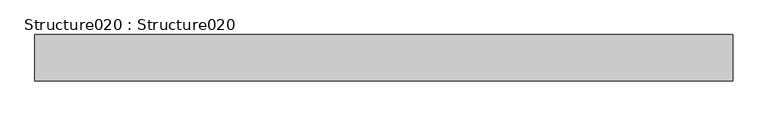
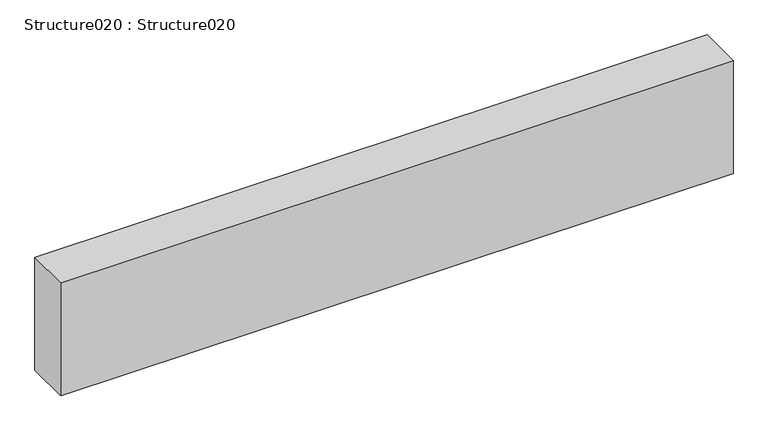
"""IFC4 building model written with IfcOpenShell, lengths in millimetres: proxy geometry, Structure020 : Structure020."""

import ifcopenshell
import ifcopenshell.guid

model = None  # the IFC model being written
_history = None  # IfcOwnerHistory: only IFC2X3 demands one
_inside = {}  # id of a spatial element -> (the spatial element, [elements in it])
_under = {}  # id of a project, library or spatial element -> (it, [spatial elements below it])
_declared = {}  # id of a project -> (the project, [libraries it declares])
_typed = {}  # id of a type object -> (the type object, [elements of that type])
_made_of = {}  # id of a material, layer set ... -> (it, [elements and type objects made of it])


def new_model(schema):
    """Start an empty IFC model of exactly this schema.

    Asked for "IFC4X3", IfcOpenShell would pick the latest addendum, in which some entities
    have other attributes; the version numbers below select the first issue.
    IFC2X3 requires an IfcOwnerHistory on every rooted entity: one is made here for all.
    """
    global model, _history
    if schema == "IFC4X3":
        model = ifcopenshell.file(schema_version=(4, 3, 0, 0))
    else:
        model = ifcopenshell.file(schema=schema)
    _inside.clear()
    _under.clear()
    _declared.clear()
    _typed.clear()
    _made_of.clear()
    _history = None
    if model.schema == "IFC2X3":
        org = make("IfcOrganization", Name="unknown")
        user = make(
            "IfcPersonAndOrganization",
            ThePerson=make("IfcPerson", FamilyName="unknown"),
            TheOrganization=org,
        )
        app = make(
            "IfcApplication",
            ApplicationDeveloper=org,
            Version="unknown",
            ApplicationFullName="unknown",
            ApplicationIdentifier="unknown",
        )
        _history = make(
            "IfcOwnerHistory",
            OwningUser=user,
            OwningApplication=app,
            ChangeAction="ADDED",
            CreationDate=0,
        )
    return model


def make(cls, **values):
    """One entity of the class cls with the attributes given. An attribute that is None is left unset."""
    return model.create_entity(
        cls, **{name: value for name, value in values.items() if value is not None}
    )


def rooted(cls, **values):
    """An entity with a GlobalId (a new one), such as an element, a storey or a relation."""
    return make(cls, GlobalId=ifcopenshell.guid.new(), OwnerHistory=_history, **values)


def si_unit(unit_type, name, prefix=None):
    """IfcSIUnit, for example si_unit("LENGTHUNIT", "METRE", prefix="MILLI")."""
    return make("IfcSIUnit", UnitType=unit_type, Prefix=prefix, Name=name)


def assignment(units):
    """IfcUnitAssignment: the units of a project."""
    return None if units is None else make("IfcUnitAssignment", Units=units)


def point(xyz):
    """IfcCartesianPoint."""
    return None if xyz is None else make("IfcCartesianPoint", Coordinates=xyz)


def direction(xyz):
    """IfcDirection."""
    return None if xyz is None else make("IfcDirection", DirectionRatios=xyz)


def frame(location, z_axis=None, x_axis=None):
    """IfcAxis2Placement3D, a coordinate frame: its origin and axes. An axis left out is left unset."""
    return make(
        "IfcAxis2Placement3D",
        Location=point(location),
        Axis=direction(z_axis),
        RefDirection=direction(x_axis),
    )


def origin():
    """The frame at (0, 0, 0) with its axes left unset."""
    return frame((0.0, 0.0, 0.0))


def place(relative_to, where):
    """IfcLocalPlacement: puts the frame where relative to a parent placement (None: the world)."""
    return make(
        "IfcLocalPlacement", PlacementRelTo=relative_to, RelativePlacement=where
    )


def context(
    kind, dimensions, precision=None, world=None, true_north=None, identifier=None
):
    """IfcGeometricRepresentationContext, for example the 3D "Model" context."""
    return make(
        "IfcGeometricRepresentationContext",
        ContextIdentifier=identifier,
        ContextType=kind,
        CoordinateSpaceDimension=dimensions,
        Precision=precision,
        WorldCoordinateSystem=world,
        TrueNorth=true_north,
    )


def project(units=None, contexts=None):
    """IfcProject with its units and contexts."""
    return rooted(
        "IfcProject",
        Name="project",
        RepresentationContexts=contexts,
        UnitsInContext=assignment(units),
    )


def spatial(cls, under=None, at=None, **own):
    """A site, building, storey or space (cls), placed at a placement, below another one or the project."""
    s = rooted(cls, ObjectPlacement=at, **own)
    if under is not None:
        _under.setdefault(under.id(), (under, []))[1].append(s)
    return s


def polyline(points):
    """IfcPolyline through the points."""
    return make("IfcPolyline", Points=[point(p) for p in points])


def outline(outer, holes=None, kind="AREA"):
    """IfcArbitraryClosedProfileDef: a profile drawn as a closed curve; with holes, ...WithVoids."""
    if holes is None:
        return make("IfcArbitraryClosedProfileDef", ProfileType=kind, OuterCurve=outer)
    return make(
        "IfcArbitraryProfileDefWithVoids",
        ProfileType=kind,
        OuterCurve=outer,
        InnerCurves=holes,
    )


def extrude(swept, where, along, depth):
    """IfcExtrudedAreaSolid: the profile swept, set in the frame where, extruded along a direction by depth."""
    return make(
        "IfcExtrudedAreaSolid",
        SweptArea=swept,
        Position=where,
        ExtrudedDirection=direction(along),
        Depth=depth,
    )


def shape(context_of_items, identifier, shape_type, items):
    """IfcShapeRepresentation: the items that make up one representation, for example the "Body"."""
    return make(
        "IfcShapeRepresentation",
        ContextOfItems=context_of_items,
        RepresentationIdentifier=identifier,
        RepresentationType=shape_type,
        Items=items,
    )


def source(mapping_origin, context_of_items, identifier, shape_type, items):
    """IfcRepresentationMap: a shape defined once, which mapped items show again and again."""
    return make(
        "IfcRepresentationMap",
        MappingOrigin=mapping_origin,
        MappedRepresentation=shape(context_of_items, identifier, shape_type, items),
    )


def transform(
    local_origin,
    x_axis=None,
    y_axis=None,
    z_axis=None,
    scale=None,
    scale2=None,
    scale3=None,
    uniform=True,
):
    """IfcCartesianTransformationOperator3D, or its non-uniform kind. x_axis, y_axis, z_axis: its Axis1, 2, 3."""
    if uniform:
        return make(
            "IfcCartesianTransformationOperator3D",
            Axis1=direction(x_axis),
            Axis2=direction(y_axis),
            LocalOrigin=point(local_origin),
            Scale=scale,
            Axis3=direction(z_axis),
        )
    return make(
        "IfcCartesianTransformationOperator3DnonUniform",
        Axis1=direction(x_axis),
        Axis2=direction(y_axis),
        LocalOrigin=point(local_origin),
        Scale=scale,
        Axis3=direction(z_axis),
        Scale2=scale2,
        Scale3=scale3,
    )


def mapped(mapping_source, mapping_target):
    """IfcMappedItem: shows the shape of a source again, moved by a transform."""
    return make(
        "IfcMappedItem", MappingSource=mapping_source, MappingTarget=mapping_target
    )


def made_of(thing, what):
    """Note that an element or type object is made of a material, layer set ...; save() writes the relation."""
    if what is not None:
        _made_of.setdefault(what.id(), (what, []))[1].append(thing)
    return thing


def element(
    cls,
    number,
    at=None,
    inside=None,
    cuts=None,
    type_object=None,
    material=None,
    context=None,
    identifier="Body",
    shape_type=None,
    held_by="IfcProductDefinitionShape",
    body=None,
    shapes=None,
    **own,
):
    """One element of the class cls, such as IfcWall. Its Tag is "e" and its number.

    at: its placement. inside: the storey or other place that contains it. cuts: it is an
    opening in that element (IfcRelVoidsElement). A single representation is given by context,
    identifier, shape_type and body (its items); several are given by shapes. held_by: the class
    of the entity that holds the representations. save() writes the other relations.
    """
    e = rooted(cls, Tag="e%d" % number, ObjectPlacement=at, **own)
    if body is not None:
        shapes = [shape(context, identifier, shape_type, body)]
    if shapes is not None:
        e.Representation = make(held_by, Representations=shapes)
    if inside is not None:
        _inside.setdefault(inside.id(), (inside, []))[1].append(e)
    if cuts is not None:
        rooted(
            "IfcRelVoidsElement", RelatingBuildingElement=cuts, RelatedOpeningElement=e
        )
    if type_object is not None:
        _typed.setdefault(type_object.id(), (type_object, []))[1].append(e)
    return made_of(e, material)


def aggregate(whole, parts):
    """IfcRelAggregates: a whole, such as a stair, and the parts it consists of."""
    return rooted("IfcRelAggregates", RelatingObject=whole, RelatedObjects=parts)


def save(model, path):
    """Write the relations noted so far, then the file.

    IfcRelAggregates (storeys below a building ...), IfcRelContainedInSpatialStructure (elements
    in a storey), IfcRelDefinesByType, IfcRelAssociatesMaterial and IfcRelDeclares: one each for
    every whole, place, type object, material and project.
    """
    for whole, parts in _under.values():
        aggregate(whole, parts)
    for where, things in _inside.values():
        rooted(
            "IfcRelContainedInSpatialStructure",
            RelatedElements=things,
            RelatingStructure=where,
        )
    for kind, things in _typed.values():
        rooted("IfcRelDefinesByType", RelatedObjects=things, RelatingType=kind)
    for what, things in _made_of.values():
        rooted("IfcRelAssociatesMaterial", RelatedObjects=things, RelatingMaterial=what)
    for by, libraries in _declared.values():
        rooted("IfcRelDeclares", RelatingContext=by, RelatedDefinitions=libraries)
    model.write(path)


def structure020_structure020_7dce29cf(model_context):
    return source(origin(), model_context, "Body", "SweptSolid", [
        extrude(outline(polyline([(14383.0178845, -5402.7175368), (14383.0178845, -5536.0675368), (12383.0178845, -5536.0675368), (12383.0178845, -5402.7175368), (14383.0178845, -5402.7175368)])), frame((0.0, 0.0, 39757.096), z_axis=(0.0, 0.0, 1.0), x_axis=(1.0, 0.0, 0.0)), (0.0, 0.0, 1.0), 355.6),
    ])


if __name__ == "__main__":
    model = new_model("IFC4")
    model_context = context("Model", 3, world=origin())
    ifc_project = project(units=[si_unit("LENGTHUNIT", "METRE", prefix="MILLI")], contexts=[model_context])
    site = spatial("IfcSite", under=ifc_project)
    building = spatial("IfcBuilding", under=site)
    placement = place(None, origin())
    structure020_structure020_shape = structure020_structure020_7dce29cf(model_context)
    element("IfcBuildingElementProxy", 1, Name="Structure020 : Structure020", ObjectType="Structure020 : Structure020", at=placement, inside=building, context=model_context, shape_type="MappedRepresentation", body=[
        mapped(structure020_structure020_shape, transform((0.0, 0.0, 0.0), x_axis=(1.0, 0.0, 0.0), y_axis=(0.0, 1.0, 0.0), z_axis=(0.0, 0.0, 1.0))),
    ])
    save(model, "model.ifc")

# Revit data of these elements
# Type "Structure020 : Structure020"
#   NameOverride = "Structure020"
# Element 1 (IfcBuildingElementProxy, "Structure020 : Structure020")
#   Materials on its faces: "STRUCTURAL MEMBER (SEE STRUCTURAL DWGS)"
# Materials
#   "STRUCTURAL MEMBER (SEE STRUCTURAL DWGS)": class "Unassigned", colour RGB 176 134 95, transparency 0, Cost = 0
